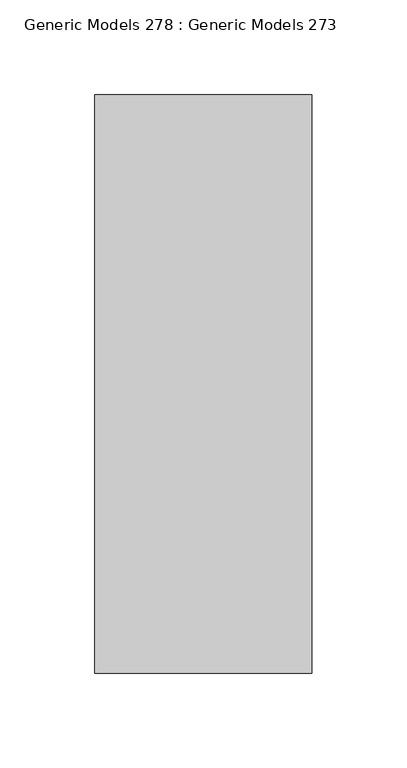
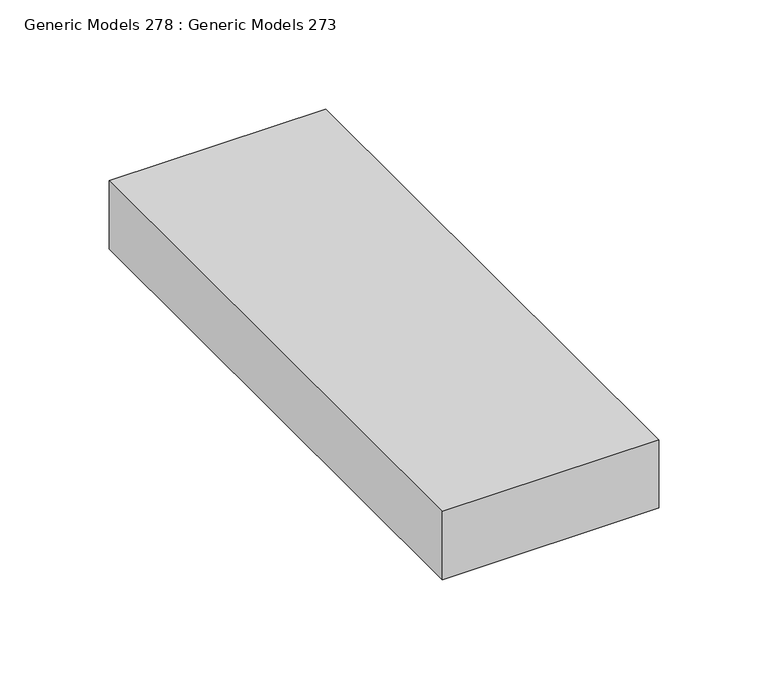
"""IFC4 building model written with IfcOpenShell, lengths in millimetres: proxy geometry, Generic Models 278 : Generic Models 273."""

from ifc_helpers import new_model, si_unit, frame, origin, place, context, project, spatial, polyline, outline, extrude, source, transform, mapped, element, save


def generic_models_278_generic_models_273_b8589f0c(model_context):
    return source(origin(), model_context, "Body", "SweptSolid", [
        extrude(outline(polyline([(1519.5401701, 4564.8872686), (1633.8199397, 4564.8872686), (1633.8199397, 4260.0872686), (1519.5401701, 4260.0872686), (1519.5401701, 4564.8872686)])), frame((0.0, 0.0, 123444.6521843), z_axis=(0.0, 0.0, 1.0), x_axis=(1.0, 0.0, 0.0)), (0.0, 0.0, 1.0), 38.1),
    ])


if __name__ == "__main__":
    model = new_model("IFC4")
    model_context = context("Model", 3, world=origin())
    ifc_project = project(units=[si_unit("LENGTHUNIT", "METRE", prefix="MILLI")], contexts=[model_context])
    site = spatial("IfcSite", under=ifc_project)
    building = spatial("IfcBuilding", under=site)
    placement = place(None, origin())
    generic_models_278_generic_models_273_shape = generic_models_278_generic_models_273_b8589f0c(model_context)
    element("IfcBuildingElementProxy", 1, Name="Generic Models 278 : Generic Models 273", ObjectType="Generic Models 278 : Generic Models 273", at=placement, inside=building, context=model_context, shape_type="MappedRepresentation", body=[
        mapped(generic_models_278_generic_models_273_shape, transform((0.0, 0.0, 0.0), x_axis=(1.0, 0.0, 0.0), y_axis=(0.0, 1.0, 0.0), z_axis=(0.0, 0.0, 1.0))),
    ])
    save(model, "model.ifc")

# Revit data of these elements
# Element 1 (IfcBuildingElementProxy, "Generic Models 278 : Generic Models 273")
#   Materials on its faces: "_TREATED BLOCKING AS REQUIRED"
# Materials
#   "_TREATED BLOCKING AS REQUIRED": class "Generic", colour RGB 177 130 114, transparency 0, Cost = 0
